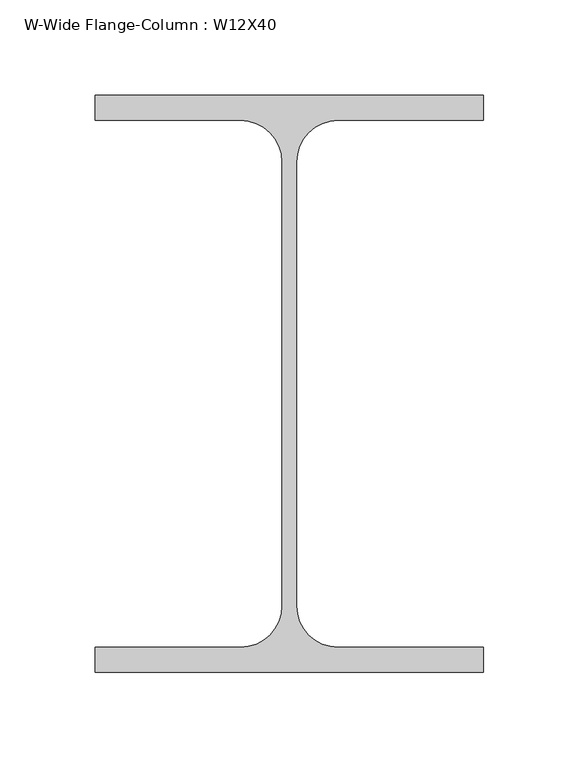
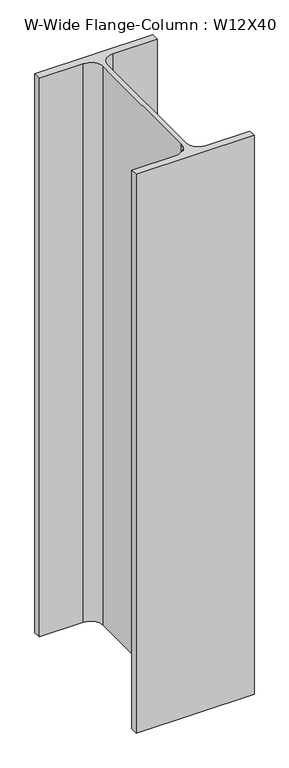
"""IFC4 building model written with IfcOpenShell, lengths in millimetres: column geometry, W-Wide Flange-Column : W12X40."""

from ifc_helpers import new_model, si_unit, point, frame, frame_2d, origin, place, context, project, spatial, polyline, circle_curve, trimmed, segment, composite_curve, outline, extrude, source, transform, mapped, element, save


def w_wide_flange_column_w12x40_63b9c914(model_context):
    return source(origin(), model_context, "Body", "SweptSolid", [
        extrude(outline(composite_curve([segment(polyline([(101.727, 151.13), (101.727, 138.049), (25.5905, 138.049)]), True, "CONTINUOUS"), segment(trimmed(circle_curve(frame_2d((25.5905, 116.205)), 21.844), [point((25.5905, 138.049))], [point((3.7465, 116.205))], True, "CARTESIAN"), True, "CONTINUOUS"), segment(polyline([(3.7465, 116.205), (3.7465, -116.205)]), True, "CONTINUOUS"), segment(trimmed(circle_curve(frame_2d((25.5905, -116.205)), 21.844), [point((3.7465, -116.205))], [point((25.5905, -138.049))], True, "CARTESIAN"), True, "CONTINUOUS"), segment(polyline([(25.5905, -138.049), (101.727, -138.049), (101.727, -151.13), (-101.727, -151.13), (-101.727, -138.049), (-25.5905, -138.049)]), True, "CONTINUOUS"), segment(trimmed(circle_curve(frame_2d((-25.5905, -116.205)), 21.844), [point((-25.5905, -138.049))], [point((-3.7465, -116.205))], True, "CARTESIAN"), True, "CONTINUOUS"), segment(polyline([(-3.7465, -116.205), (-3.7465, 116.205)]), True, "CONTINUOUS"), segment(trimmed(circle_curve(frame_2d((-25.5905, 116.205)), 21.844), [point((-3.7465, 116.205))], [point((-25.5905, 138.049))], True, "CARTESIAN"), True, "CONTINUOUS"), segment(polyline([(-25.5905, 138.049), (-101.727, 138.049), (-101.727, 151.13), (101.727, 151.13)]), True, "CONTINUOUS")], self_intersect=False)), frame((0.0, 0.0, 23317.2), z_axis=(0.0, 0.0, 1.0), x_axis=(1.0, 0.0, 0.0)), (0.0, 0.0, 1.0), 1018.5796875),
    ])


if __name__ == "__main__":
    model = new_model("IFC4")
    model_context = context("Model", 3, world=origin())
    ifc_project = project(units=[si_unit("LENGTHUNIT", "METRE", prefix="MILLI")], contexts=[model_context])
    site = spatial("IfcSite", under=ifc_project)
    building = spatial("IfcBuilding", under=site)
    placement = place(None, origin())
    w_wide_flange_column_w12x40_shape = w_wide_flange_column_w12x40_63b9c914(model_context)
    element("IfcColumn", 1, ObjectType="W-Wide Flange-Column : W12X40", at=placement, inside=building, context=model_context, shape_type="MappedRepresentation", body=[
        mapped(w_wide_flange_column_w12x40_shape, transform((0.0, 0.0, 0.0), x_axis=(1.0, 0.0, 0.0), y_axis=(0.0, 1.0, 0.0), z_axis=(0.0, 0.0, 1.0))),
    ])
    save(model, "model.ifc")

# Revit data of these elements
# Type "W-Wide Flange-Column : W12X40"
#   Assembly Code = "B10"
#   W = 40
#   bf = 0' - 8.01"
#   d = 0' - 11.9"
#   k = 0' - 1 3/8"
#   kr = 0' - 0.86"
#   tf = 0' - 0.515"
#   tw = 0' - 0.295"
#   A = 0.08125 SF
#   Structural Material [instance default] = Steel ASTM A992
# Element 1 (IfcColumn, "W-Wide Flange-Column : W12X40")
#   Materials on its faces: "Steel ASTM A992"
# Materials
#   "Steel ASTM A992": class "Metal", colour RGB 199 199 199, transparency 0, Description = "Structural steel 50ksi", Cost = 0
